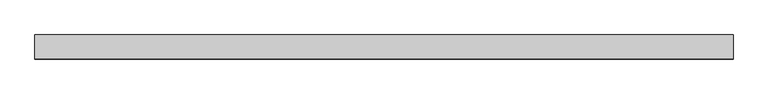
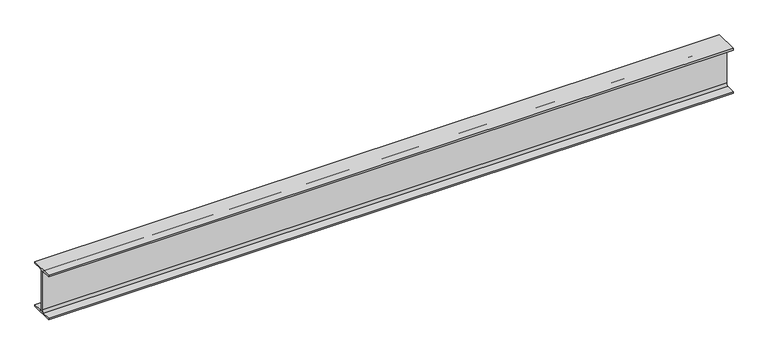
"""IFC4 building model written with IfcOpenShell, lengths in millimetres: beam geometry, 0912_Steel Framing_H-KSD3502 : H_SB_ASB_H-250x125x6x9."""

from ifc_helpers import new_model, si_unit, point, frame, frame_2d, origin, place, context, project, spatial, polyline, circle_curve, trimmed, segment, composite_curve, outline, extrude, source, transform, mapped, element, save


def beam_267930f0(model_context):
    return source(origin(), model_context, "Body", "SweptSolid", [
        extrude(outline(composite_curve([segment(polyline([(62.5, -116.0), (62.5, -125.0), (-62.5, -125.0), (-62.5, -116.0), (-15.0, -116.0)]), True, "CONTINUOUS"), segment(trimmed(circle_curve(frame_2d((-15.0, -104.0)), 12.0), [point((-15.0, -116.0))], [point((-3.0, -104.0))], True, "CARTESIAN"), True, "CONTINUOUS"), segment(polyline([(-3.0, -104.0), (-3.0, 104.0)]), True, "CONTINUOUS"), segment(trimmed(circle_curve(frame_2d((-15.0, 104.0)), 12.0), [point((-3.0, 104.0))], [point((-15.0, 116.0))], True, "CARTESIAN"), True, "CONTINUOUS"), segment(polyline([(-15.0, 116.0), (-62.5, 116.0), (-62.5, 125.0), (62.5, 125.0), (62.5, 116.0), (15.0, 116.0)]), True, "CONTINUOUS"), segment(trimmed(circle_curve(frame_2d((15.0, 104.0)), 12.0), [point((15.0, 116.0))], [point((3.0, 104.0))], True, "CARTESIAN"), True, "CONTINUOUS"), segment(polyline([(3.0, 104.0), (3.0, -104.0)]), True, "CONTINUOUS"), segment(trimmed(circle_curve(frame_2d((15.0, -104.0)), 12.0), [point((3.0, -104.0))], [point((15.0, -116.0))], True, "CARTESIAN"), True, "CONTINUOUS"), segment(polyline([(15.0, -116.0), (62.5, -116.0)]), True, "CONTINUOUS")], self_intersect=False)), frame((-1904.8, 0.0, 0.0), z_axis=(1.0, 0.0, 0.0), x_axis=(0.0, 1.0, 0.0)), (0.0, 0.0, 1.0), 3623.1833333),
    ])


if __name__ == "__main__":
    model = new_model("IFC4")
    model_context = context("Model", 3, world=origin())
    ifc_project = project(units=[si_unit("LENGTHUNIT", "METRE", prefix="MILLI")], contexts=[model_context])
    site = spatial("IfcSite", under=ifc_project)
    building = spatial("IfcBuilding", under=site)
    placement = place(None, origin())
    beam_shape = beam_267930f0(model_context)
    element("IfcBeam", 1, ObjectType="0912_Steel Framing_H-KSD3502 : H_SB_ASB_H-250x125x6x9", at=placement, inside=building, context=model_context, shape_type="MappedRepresentation", body=[
        mapped(beam_shape, transform((0.0, 0.0, 0.0), x_axis=(1.0, 0.0, 0.0), y_axis=(0.0, 1.0, 0.0), z_axis=(0.0, 0.0, 1.0))),
    ])
    save(model, "model.ifc")

# Revit data of these elements
# Type "0912_Steel Framing_H-KSD3502 : H_SB_ASB_H-250x125x6x9"
#   H_WM Code_1 = "S01AA003-00001 | Main Steel Structure Fabrication Work | Shelter/Building | Light Steel - Standard (30KG/M>Weight) | Material: (   )"
#   H_WM Code_2 = "S03AA029-00001 | Main Steel Structure Erection Work | Shelter/Building | Light Steel (30KG/M>Weight) | Material: (   )"
#   H_WM Code_3 = "S01AA010-00001 | Main Steel Structure Fabrication Work | Shelter/Building | Steel Painting/Coating | for Non-Fireproofed Steel Surface, Surface Preparation, Primer, Second & Final Coat | Material: (   )"
#   H_Q'ty Cal Type Tag = "SB-Q2"
#   Width = 12.5 cm
#   Web Thickness = 0.6 cm
#   Web Fillet = 1.2 cm
#   Warping Constant = 42539.8 cm⁶
#   W = 0
#   Torsional Moment of Inertia = 7.8102 cm⁴
#   Section Area = 37.66 cm²
#   Plastic Modulus weak axis = 73.1 cm³
#   Plastic Modulus strong axis = 366.0 cm³
#   Perimeter = 0.97 m²/m
#   Nominal Weight = 29.60 kgf/m
#   Moment of Inertia weak axis = 294.00 cm⁴
#   Moment of Inertia strong axis = 4050.00 cm⁴
#   Height = 25.0 cm
#   Flange Thickness = 0.9 cm
#   Elastic Modulus weak axis = 47.0 cm³
#   Elastic Modulus strong axis = 324.0 cm³
#   Centroid Vertical = 12.5 cm
#   Centroid Horizontal = 6.25 cm
#   Ix = 40500000
#   Length [instance default] = 1.5240 m
#   Zx = 366000
#   b = 0.1250 m
#   h = 0.2500 m
#   r = 0.0120 m
#   s = 0.0060 m
#   t = 0.0090 m
#   A = 0.003766 m²
#   Structural Material [instance default] = Steel, 45-345
#   Assembly Code = ""
# Element 1 (IfcBeam, "0912_Steel Framing_H-KSD3502 : H_SB_ASB_H-250x125x6x9")
#   Structural Material = none
# Materials
#   "Steel, 45-345": class "Metal", colour RGB 189 187 185, transparency 0, Description = "Steel 345 MPa", Cost = 0
